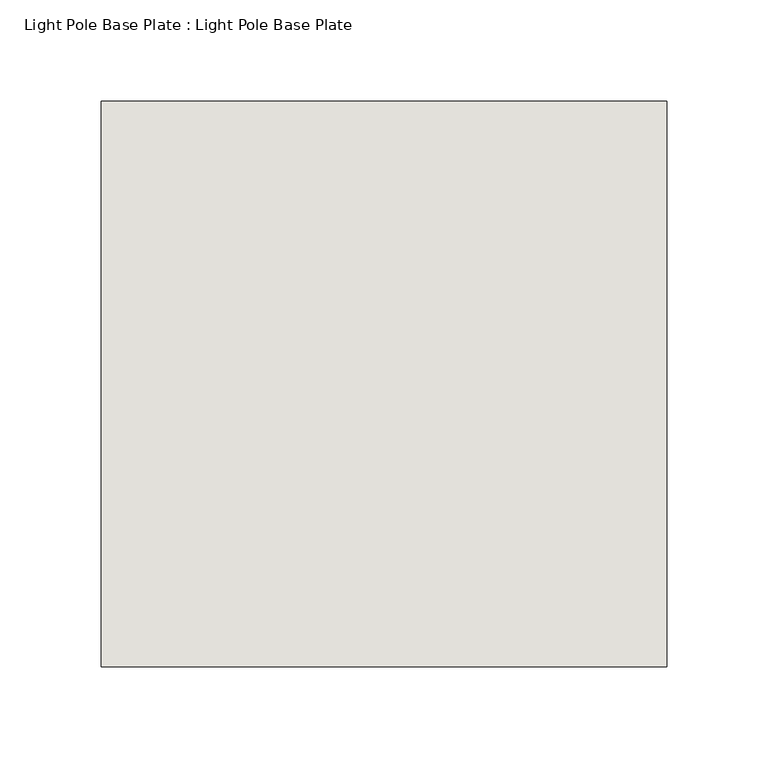
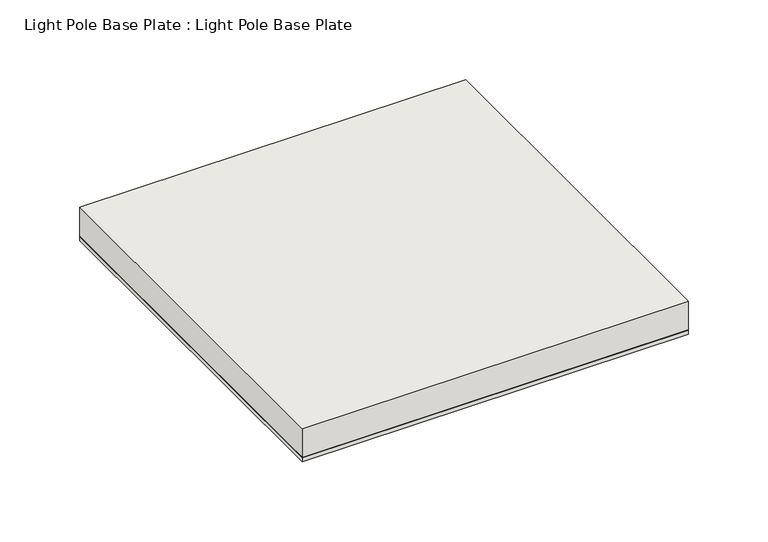
"""IFC4 building model written with IfcOpenShell, lengths in millimetres: wall geometry, Light Pole Base Plate : Light Pole Base Plate."""

from ifc_helpers import new_model, si_unit, frame, origin, place, context, project, spatial, polyline, outline, extrude, source, transform, mapped, element, save


def light_pole_base_plate_light_pole_base_plate_e22e9f66(model_context):
    return source(origin(), model_context, "Body", "SweptSolid", [
        extrude(outline(polyline([(40225.6625, 731.8375), (40505.0625, 731.8375), (40505.0625, 452.4375), (40225.6625, 452.4375), (40225.6625, 731.8375)])), frame((0.0, 0.0, 762.0), z_axis=(0.0, 0.0, 1.0), x_axis=(1.0, 0.0, 0.0)), (0.0, 0.0, 1.0), 3.175),
        extrude(outline(polyline([(40225.6625, 731.8375), (40505.0625, 731.8375), (40505.0625, 452.4375), (40225.6625, 452.4375), (40225.6625, 731.8375)])), frame((0.0, 0.0, 765.175), z_axis=(0.0, 0.0, 1.0), x_axis=(1.0, 0.0, 0.0)), (0.0, 0.0, 1.0), 22.225),
    ])


if __name__ == "__main__":
    model = new_model("IFC4")
    model_context = context("Model", 3, world=origin())
    ifc_project = project(units=[si_unit("LENGTHUNIT", "METRE", prefix="MILLI")], contexts=[model_context])
    site = spatial("IfcSite", under=ifc_project)
    building = spatial("IfcBuilding", under=site)
    placement = place(None, origin())
    light_pole_base_plate_light_pole_base_plate_shape = light_pole_base_plate_light_pole_base_plate_e22e9f66(model_context)
    element("IfcWall", 1, ObjectType="Light Pole Base Plate : Light Pole Base Plate", at=placement, inside=building, context=model_context, shape_type="MappedRepresentation", body=[
        mapped(light_pole_base_plate_light_pole_base_plate_shape, transform((0.0, 0.0, 0.0), x_axis=(1.0, 0.0, 0.0), y_axis=(0.0, 1.0, 0.0), z_axis=(0.0, 0.0, 1.0))),
    ])
    save(model, "model.ifc")

# Revit data of these elements
# Element 1 (IfcWall, "Light Pole Base Plate : Light Pole Base Plate")
#   Materials on its faces: "SHIMS FOR PROPER VENTILATION", "STEEL BASE PLATE"
# Materials
#   "SHIMS FOR PROPER VENTILATION": class "Miscellaneous", colour RGB 104 103 100, transparency 0, Cost = 0
#   "STEEL BASE PLATE": class "Metal", colour RGB 199 199 199, transparency 0, Description = "Carbon steel", Cost = 0
